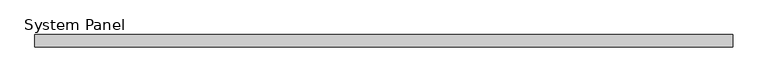
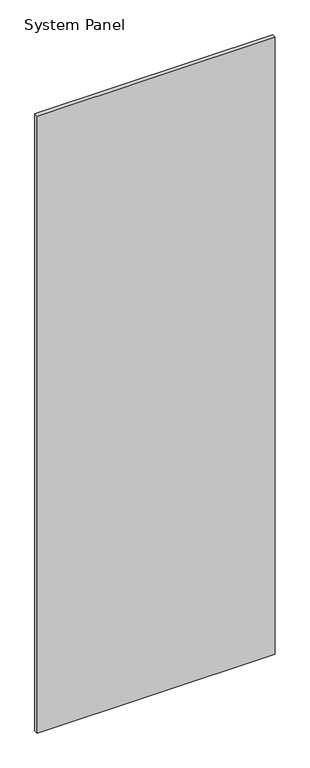
"""IFC4 building model written with IfcOpenShell, lengths in millimetres: plate geometry, System Panel : WWm-Glass-20mm-10mmOffset."""

from ifc_helpers import new_model, si_unit, origin, origin_with_axes, place, context, project, spatial, polyline, outline, extrude, source, transform, mapped, element, save


def system_panel_9caeb6a4(model_context):
    return source(origin(), model_context, "Body", "SweptSolid", [
        extrude(outline(polyline([(575.0, 0.0), (-575.0, 0.0), (-575.0, 20.0), (575.0, 20.0), (575.0, 0.0)])), origin_with_axes(), (0.0, 0.0, 1.0), 3150.0),
    ])


if __name__ == "__main__":
    model = new_model("IFC4")
    model_context = context("Model", 3, world=origin())
    ifc_project = project(units=[si_unit("LENGTHUNIT", "METRE", prefix="MILLI")], contexts=[model_context])
    site = spatial("IfcSite", under=ifc_project)
    building = spatial("IfcBuilding", under=site)
    placement = place(None, origin())
    system_panel_shape = system_panel_9caeb6a4(model_context)
    element("IfcPlate", 1, ObjectType="System Panel : WWm-Glass-20mm-10mmOffset", at=placement, inside=building, context=model_context, shape_type="MappedRepresentation", body=[
        mapped(system_panel_shape, transform((0.0, 0.0, 0.0), x_axis=(1.0, 0.0, 0.0), y_axis=(0.0, 1.0, 0.0), z_axis=(0.0, 0.0, 1.0))),
    ])
    save(model, "model.ifc")

# Revit data of these elements
# Type "System Panel : WWm-Glass-20mm-10mmOffset"
#   Finish = ""
# Element 1 (IfcPlate, "System Panel : WWm-Glass-20mm-10mmOffset")
#   Materials on its faces: "WW-EC-GL-Storefront"
# Materials
#   "WW-EC-GL-Storefront": class "Glass", colour RGB 236 240 239, transparency 0.85, Description = "Storefront Glass", Cost = 0
